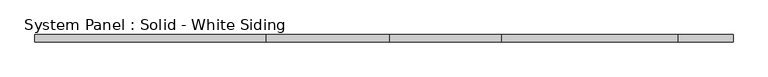
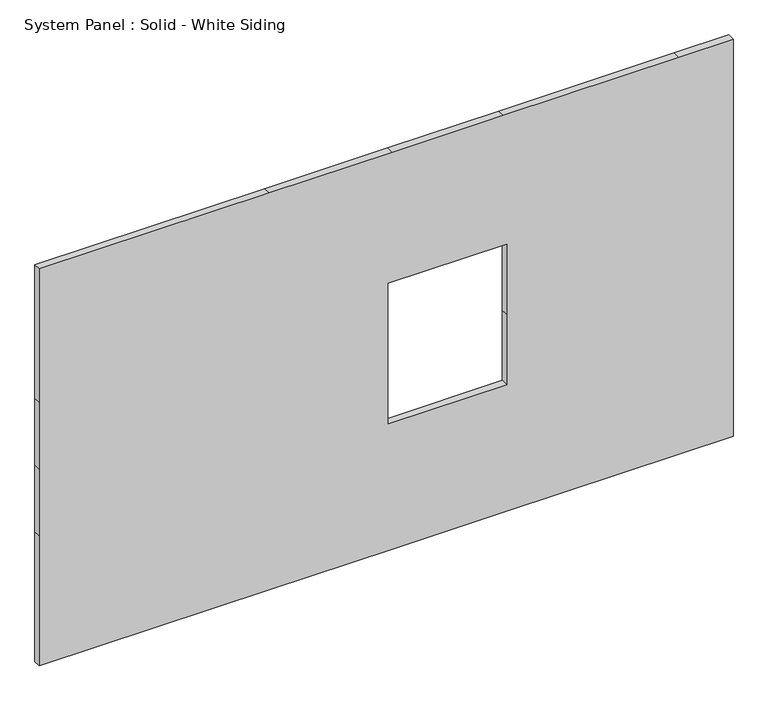
"""IFC4 building model written with IfcOpenShell, lengths in millimetres: plate geometry, System Panel : Solid - White Siding."""

import ifcopenshell
import ifcopenshell.guid

model = None  # the IFC model being written
_history = None  # IfcOwnerHistory: only IFC2X3 demands one
_inside = {}  # id of a spatial element -> (the spatial element, [elements in it])
_under = {}  # id of a project, library or spatial element -> (it, [spatial elements below it])
_declared = {}  # id of a project -> (the project, [libraries it declares])
_typed = {}  # id of a type object -> (the type object, [elements of that type])
_made_of = {}  # id of a material, layer set ... -> (it, [elements and type objects made of it])


def new_model(schema):
    """Start an empty IFC model of exactly this schema.

    Asked for "IFC4X3", IfcOpenShell would pick the latest addendum, in which some entities
    have other attributes; the version numbers below select the first issue.
    IFC2X3 requires an IfcOwnerHistory on every rooted entity: one is made here for all.
    """
    global model, _history
    if schema == "IFC4X3":
        model = ifcopenshell.file(schema_version=(4, 3, 0, 0))
    else:
        model = ifcopenshell.file(schema=schema)
    _inside.clear()
    _under.clear()
    _declared.clear()
    _typed.clear()
    _made_of.clear()
    _history = None
    if model.schema == "IFC2X3":
        org = make("IfcOrganization", Name="unknown")
        user = make(
            "IfcPersonAndOrganization",
            ThePerson=make("IfcPerson", FamilyName="unknown"),
            TheOrganization=org,
        )
        app = make(
            "IfcApplication",
            ApplicationDeveloper=org,
            Version="unknown",
            ApplicationFullName="unknown",
            ApplicationIdentifier="unknown",
        )
        _history = make(
            "IfcOwnerHistory",
            OwningUser=user,
            OwningApplication=app,
            ChangeAction="ADDED",
            CreationDate=0,
        )
    return model


def make(cls, **values):
    """One entity of the class cls with the attributes given. An attribute that is None is left unset."""
    return model.create_entity(
        cls, **{name: value for name, value in values.items() if value is not None}
    )


def rooted(cls, **values):
    """An entity with a GlobalId (a new one), such as an element, a storey or a relation."""
    return make(cls, GlobalId=ifcopenshell.guid.new(), OwnerHistory=_history, **values)


def si_unit(unit_type, name, prefix=None):
    """IfcSIUnit, for example si_unit("LENGTHUNIT", "METRE", prefix="MILLI")."""
    return make("IfcSIUnit", UnitType=unit_type, Prefix=prefix, Name=name)


def assignment(units):
    """IfcUnitAssignment: the units of a project."""
    return None if units is None else make("IfcUnitAssignment", Units=units)


def point(xyz):
    """IfcCartesianPoint."""
    return None if xyz is None else make("IfcCartesianPoint", Coordinates=xyz)


def direction(xyz):
    """IfcDirection."""
    return None if xyz is None else make("IfcDirection", DirectionRatios=xyz)


def frame(location, z_axis=None, x_axis=None):
    """IfcAxis2Placement3D, a coordinate frame: its origin and axes. An axis left out is left unset."""
    return make(
        "IfcAxis2Placement3D",
        Location=point(location),
        Axis=direction(z_axis),
        RefDirection=direction(x_axis),
    )


def origin():
    """The frame at (0, 0, 0) with its axes left unset."""
    return frame((0.0, 0.0, 0.0))


def place(relative_to, where):
    """IfcLocalPlacement: puts the frame where relative to a parent placement (None: the world)."""
    return make(
        "IfcLocalPlacement", PlacementRelTo=relative_to, RelativePlacement=where
    )


def context(
    kind, dimensions, precision=None, world=None, true_north=None, identifier=None
):
    """IfcGeometricRepresentationContext, for example the 3D "Model" context."""
    return make(
        "IfcGeometricRepresentationContext",
        ContextIdentifier=identifier,
        ContextType=kind,
        CoordinateSpaceDimension=dimensions,
        Precision=precision,
        WorldCoordinateSystem=world,
        TrueNorth=true_north,
    )


def project(units=None, contexts=None):
    """IfcProject with its units and contexts."""
    return rooted(
        "IfcProject",
        Name="project",
        RepresentationContexts=contexts,
        UnitsInContext=assignment(units),
    )


def spatial(cls, under=None, at=None, **own):
    """A site, building, storey or space (cls), placed at a placement, below another one or the project."""
    s = rooted(cls, ObjectPlacement=at, **own)
    if under is not None:
        _under.setdefault(under.id(), (under, []))[1].append(s)
    return s


def polyline(points):
    """IfcPolyline through the points."""
    return make("IfcPolyline", Points=[point(p) for p in points])


def outline(outer, holes=None, kind="AREA"):
    """IfcArbitraryClosedProfileDef: a profile drawn as a closed curve; with holes, ...WithVoids."""
    if holes is None:
        return make("IfcArbitraryClosedProfileDef", ProfileType=kind, OuterCurve=outer)
    return make(
        "IfcArbitraryProfileDefWithVoids",
        ProfileType=kind,
        OuterCurve=outer,
        InnerCurves=holes,
    )


def extrude(swept, where, along, depth):
    """IfcExtrudedAreaSolid: the profile swept, set in the frame where, extruded along a direction by depth."""
    return make(
        "IfcExtrudedAreaSolid",
        SweptArea=swept,
        Position=where,
        ExtrudedDirection=direction(along),
        Depth=depth,
    )


def shape(context_of_items, identifier, shape_type, items):
    """IfcShapeRepresentation: the items that make up one representation, for example the "Body"."""
    return make(
        "IfcShapeRepresentation",
        ContextOfItems=context_of_items,
        RepresentationIdentifier=identifier,
        RepresentationType=shape_type,
        Items=items,
    )


def source(mapping_origin, context_of_items, identifier, shape_type, items):
    """IfcRepresentationMap: a shape defined once, which mapped items show again and again."""
    return make(
        "IfcRepresentationMap",
        MappingOrigin=mapping_origin,
        MappedRepresentation=shape(context_of_items, identifier, shape_type, items),
    )


def transform(
    local_origin,
    x_axis=None,
    y_axis=None,
    z_axis=None,
    scale=None,
    scale2=None,
    scale3=None,
    uniform=True,
):
    """IfcCartesianTransformationOperator3D, or its non-uniform kind. x_axis, y_axis, z_axis: its Axis1, 2, 3."""
    if uniform:
        return make(
            "IfcCartesianTransformationOperator3D",
            Axis1=direction(x_axis),
            Axis2=direction(y_axis),
            LocalOrigin=point(local_origin),
            Scale=scale,
            Axis3=direction(z_axis),
        )
    return make(
        "IfcCartesianTransformationOperator3DnonUniform",
        Axis1=direction(x_axis),
        Axis2=direction(y_axis),
        LocalOrigin=point(local_origin),
        Scale=scale,
        Axis3=direction(z_axis),
        Scale2=scale2,
        Scale3=scale3,
    )


def mapped(mapping_source, mapping_target):
    """IfcMappedItem: shows the shape of a source again, moved by a transform."""
    return make(
        "IfcMappedItem", MappingSource=mapping_source, MappingTarget=mapping_target
    )


def made_of(thing, what):
    """Note that an element or type object is made of a material, layer set ...; save() writes the relation."""
    if what is not None:
        _made_of.setdefault(what.id(), (what, []))[1].append(thing)
    return thing


def element(
    cls,
    number,
    at=None,
    inside=None,
    cuts=None,
    type_object=None,
    material=None,
    context=None,
    identifier="Body",
    shape_type=None,
    held_by="IfcProductDefinitionShape",
    body=None,
    shapes=None,
    **own,
):
    """One element of the class cls, such as IfcWall. Its Tag is "e" and its number.

    at: its placement. inside: the storey or other place that contains it. cuts: it is an
    opening in that element (IfcRelVoidsElement). A single representation is given by context,
    identifier, shape_type and body (its items); several are given by shapes. held_by: the class
    of the entity that holds the representations. save() writes the other relations.
    """
    e = rooted(cls, Tag="e%d" % number, ObjectPlacement=at, **own)
    if body is not None:
        shapes = [shape(context, identifier, shape_type, body)]
    if shapes is not None:
        e.Representation = make(held_by, Representations=shapes)
    if inside is not None:
        _inside.setdefault(inside.id(), (inside, []))[1].append(e)
    if cuts is not None:
        rooted(
            "IfcRelVoidsElement", RelatingBuildingElement=cuts, RelatedOpeningElement=e
        )
    if type_object is not None:
        _typed.setdefault(type_object.id(), (type_object, []))[1].append(e)
    return made_of(e, material)


def aggregate(whole, parts):
    """IfcRelAggregates: a whole, such as a stair, and the parts it consists of."""
    return rooted("IfcRelAggregates", RelatingObject=whole, RelatedObjects=parts)


def save(model, path):
    """Write the relations noted so far, then the file.

    IfcRelAggregates (storeys below a building ...), IfcRelContainedInSpatialStructure (elements
    in a storey), IfcRelDefinesByType, IfcRelAssociatesMaterial and IfcRelDeclares: one each for
    every whole, place, type object, material and project.
    """
    for whole, parts in _under.values():
        aggregate(whole, parts)
    for where, things in _inside.values():
        rooted(
            "IfcRelContainedInSpatialStructure",
            RelatedElements=things,
            RelatingStructure=where,
        )
    for kind, things in _typed.values():
        rooted("IfcRelDefinesByType", RelatedObjects=things, RelatingType=kind)
    for what, things in _made_of.values():
        rooted("IfcRelAssociatesMaterial", RelatedObjects=things, RelatingMaterial=what)
    for by, libraries in _declared.values():
        rooted("IfcRelDeclares", RelatingContext=by, RelatedDefinitions=libraries)
    model.write(path)


def system_panel_solid_white_siding_b96ba671(model_context):
    return source(origin(), model_context, "Body", "SweptSolid", [
        extrude(outline(polyline([(0.0, -2997.2), (0.0, -1009.65), (0.0, 50.8), (0.0, 1009.65), (0.0, 2527.3), (0.0, 2997.2), (1187.45, 2997.2), (1797.05, 2997.2), (2406.65, 2997.2), (3625.85, 2997.2), (3625.85, 2527.3), (3625.85, 1009.65), (3625.85, 50.8), (3625.85, -1009.65), (3625.85, -2997.2), (2406.65, -2997.2), (1797.05, -2997.2), (1187.45, -2997.2), (0.0, -2997.2)]), holes=[polyline([(1155.7, 1041.4), (1155.7, 19.05), (1797.05, 19.05), (2438.4, 19.05), (2438.4, 1041.4), (1797.05, 1041.4), (1155.7, 1041.4)])]), frame((0.0, -44.45, 0.0), z_axis=(0.0, 1.0, 0.0), x_axis=(0.0, 0.0, 1.0)), (0.0, 0.0, 1.0), 63.5),
    ])


if __name__ == "__main__":
    model = new_model("IFC4")
    model_context = context("Model", 3, world=origin())
    ifc_project = project(units=[si_unit("LENGTHUNIT", "METRE", prefix="MILLI")], contexts=[model_context])
    site = spatial("IfcSite", under=ifc_project)
    building = spatial("IfcBuilding", under=site)
    placement = place(None, origin())
    system_panel_solid_white_siding_shape = system_panel_solid_white_siding_b96ba671(model_context)
    element("IfcPlate", 1, ObjectType="System Panel : Solid - White Siding", at=placement, inside=building, context=model_context, shape_type="MappedRepresentation", body=[
        mapped(system_panel_solid_white_siding_shape, transform((0.0, 0.0, 0.0), x_axis=(1.0, 0.0, 0.0), y_axis=(0.0, 1.0, 0.0), z_axis=(0.0, 0.0, 1.0))),
    ])
    save(model, "model.ifc")

# Revit data of these elements
# Element 1 (IfcPlate, "System Panel : Solid - White Siding")
#   Materials on its faces: "White Siding"
# Materials
#   "White Siding": class "Unassigned", colour RGB 255 255 255, transparency 0
